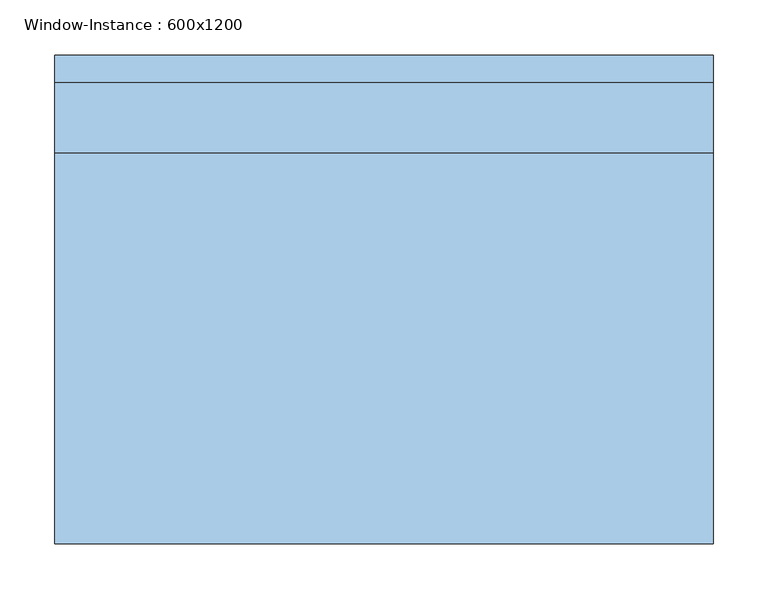
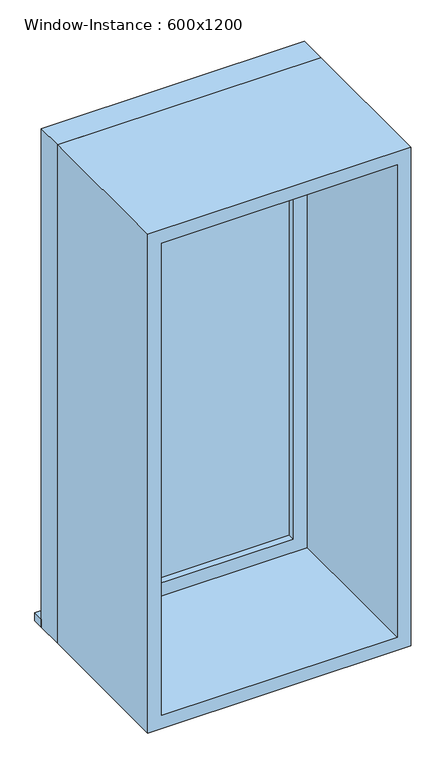
"""IFC4 building model written with IfcOpenShell, lengths in millimetres: window geometry, Window-Instance : 600x1200."""

import ifcopenshell
import ifcopenshell.guid

model = None  # the IFC model being written
_history = None  # IfcOwnerHistory: only IFC2X3 demands one
_inside = {}  # id of a spatial element -> (the spatial element, [elements in it])
_under = {}  # id of a project, library or spatial element -> (it, [spatial elements below it])
_declared = {}  # id of a project -> (the project, [libraries it declares])
_typed = {}  # id of a type object -> (the type object, [elements of that type])
_made_of = {}  # id of a material, layer set ... -> (it, [elements and type objects made of it])


def new_model(schema):
    """Start an empty IFC model of exactly this schema.

    Asked for "IFC4X3", IfcOpenShell would pick the latest addendum, in which some entities
    have other attributes; the version numbers below select the first issue.
    IFC2X3 requires an IfcOwnerHistory on every rooted entity: one is made here for all.
    """
    global model, _history
    if schema == "IFC4X3":
        model = ifcopenshell.file(schema_version=(4, 3, 0, 0))
    else:
        model = ifcopenshell.file(schema=schema)
    _inside.clear()
    _under.clear()
    _declared.clear()
    _typed.clear()
    _made_of.clear()
    _history = None
    if model.schema == "IFC2X3":
        org = make("IfcOrganization", Name="unknown")
        user = make(
            "IfcPersonAndOrganization",
            ThePerson=make("IfcPerson", FamilyName="unknown"),
            TheOrganization=org,
        )
        app = make(
            "IfcApplication",
            ApplicationDeveloper=org,
            Version="unknown",
            ApplicationFullName="unknown",
            ApplicationIdentifier="unknown",
        )
        _history = make(
            "IfcOwnerHistory",
            OwningUser=user,
            OwningApplication=app,
            ChangeAction="ADDED",
            CreationDate=0,
        )
    return model


def make(cls, **values):
    """One entity of the class cls with the attributes given. An attribute that is None is left unset."""
    return model.create_entity(
        cls, **{name: value for name, value in values.items() if value is not None}
    )


def rooted(cls, **values):
    """An entity with a GlobalId (a new one), such as an element, a storey or a relation."""
    return make(cls, GlobalId=ifcopenshell.guid.new(), OwnerHistory=_history, **values)


def si_unit(unit_type, name, prefix=None):
    """IfcSIUnit, for example si_unit("LENGTHUNIT", "METRE", prefix="MILLI")."""
    return make("IfcSIUnit", UnitType=unit_type, Prefix=prefix, Name=name)


def assignment(units):
    """IfcUnitAssignment: the units of a project."""
    return None if units is None else make("IfcUnitAssignment", Units=units)


def point(xyz):
    """IfcCartesianPoint."""
    return None if xyz is None else make("IfcCartesianPoint", Coordinates=xyz)


def direction(xyz):
    """IfcDirection."""
    return None if xyz is None else make("IfcDirection", DirectionRatios=xyz)


def frame(location, z_axis=None, x_axis=None):
    """IfcAxis2Placement3D, a coordinate frame: its origin and axes. An axis left out is left unset."""
    return make(
        "IfcAxis2Placement3D",
        Location=point(location),
        Axis=direction(z_axis),
        RefDirection=direction(x_axis),
    )


def origin():
    """The frame at (0, 0, 0) with its axes left unset."""
    return frame((0.0, 0.0, 0.0))


def place(relative_to, where):
    """IfcLocalPlacement: puts the frame where relative to a parent placement (None: the world)."""
    return make(
        "IfcLocalPlacement", PlacementRelTo=relative_to, RelativePlacement=where
    )


def context(
    kind, dimensions, precision=None, world=None, true_north=None, identifier=None
):
    """IfcGeometricRepresentationContext, for example the 3D "Model" context."""
    return make(
        "IfcGeometricRepresentationContext",
        ContextIdentifier=identifier,
        ContextType=kind,
        CoordinateSpaceDimension=dimensions,
        Precision=precision,
        WorldCoordinateSystem=world,
        TrueNorth=true_north,
    )


def project(units=None, contexts=None):
    """IfcProject with its units and contexts."""
    return rooted(
        "IfcProject",
        Name="project",
        RepresentationContexts=contexts,
        UnitsInContext=assignment(units),
    )


def spatial(cls, under=None, at=None, **own):
    """A site, building, storey or space (cls), placed at a placement, below another one or the project."""
    s = rooted(cls, ObjectPlacement=at, **own)
    if under is not None:
        _under.setdefault(under.id(), (under, []))[1].append(s)
    return s


def polyline(points):
    """IfcPolyline through the points."""
    return make("IfcPolyline", Points=[point(p) for p in points])


def outline(outer, holes=None, kind="AREA"):
    """IfcArbitraryClosedProfileDef: a profile drawn as a closed curve; with holes, ...WithVoids."""
    if holes is None:
        return make("IfcArbitraryClosedProfileDef", ProfileType=kind, OuterCurve=outer)
    return make(
        "IfcArbitraryProfileDefWithVoids",
        ProfileType=kind,
        OuterCurve=outer,
        InnerCurves=holes,
    )


def extrude(swept, where, along, depth):
    """IfcExtrudedAreaSolid: the profile swept, set in the frame where, extruded along a direction by depth."""
    return make(
        "IfcExtrudedAreaSolid",
        SweptArea=swept,
        Position=where,
        ExtrudedDirection=direction(along),
        Depth=depth,
    )


def shape(context_of_items, identifier, shape_type, items):
    """IfcShapeRepresentation: the items that make up one representation, for example the "Body"."""
    return make(
        "IfcShapeRepresentation",
        ContextOfItems=context_of_items,
        RepresentationIdentifier=identifier,
        RepresentationType=shape_type,
        Items=items,
    )


def source(mapping_origin, context_of_items, identifier, shape_type, items):
    """IfcRepresentationMap: a shape defined once, which mapped items show again and again."""
    return make(
        "IfcRepresentationMap",
        MappingOrigin=mapping_origin,
        MappedRepresentation=shape(context_of_items, identifier, shape_type, items),
    )


def transform(
    local_origin,
    x_axis=None,
    y_axis=None,
    z_axis=None,
    scale=None,
    scale2=None,
    scale3=None,
    uniform=True,
):
    """IfcCartesianTransformationOperator3D, or its non-uniform kind. x_axis, y_axis, z_axis: its Axis1, 2, 3."""
    if uniform:
        return make(
            "IfcCartesianTransformationOperator3D",
            Axis1=direction(x_axis),
            Axis2=direction(y_axis),
            LocalOrigin=point(local_origin),
            Scale=scale,
            Axis3=direction(z_axis),
        )
    return make(
        "IfcCartesianTransformationOperator3DnonUniform",
        Axis1=direction(x_axis),
        Axis2=direction(y_axis),
        LocalOrigin=point(local_origin),
        Scale=scale,
        Axis3=direction(z_axis),
        Scale2=scale2,
        Scale3=scale3,
    )


def mapped(mapping_source, mapping_target):
    """IfcMappedItem: shows the shape of a source again, moved by a transform."""
    return make(
        "IfcMappedItem", MappingSource=mapping_source, MappingTarget=mapping_target
    )


def made_of(thing, what):
    """Note that an element or type object is made of a material, layer set ...; save() writes the relation."""
    if what is not None:
        _made_of.setdefault(what.id(), (what, []))[1].append(thing)
    return thing


def element(
    cls,
    number,
    at=None,
    inside=None,
    cuts=None,
    type_object=None,
    material=None,
    context=None,
    identifier="Body",
    shape_type=None,
    held_by="IfcProductDefinitionShape",
    body=None,
    shapes=None,
    **own,
):
    """One element of the class cls, such as IfcWall. Its Tag is "e" and its number.

    at: its placement. inside: the storey or other place that contains it. cuts: it is an
    opening in that element (IfcRelVoidsElement). A single representation is given by context,
    identifier, shape_type and body (its items); several are given by shapes. held_by: the class
    of the entity that holds the representations. save() writes the other relations.
    """
    e = rooted(cls, Tag="e%d" % number, ObjectPlacement=at, **own)
    if body is not None:
        shapes = [shape(context, identifier, shape_type, body)]
    if shapes is not None:
        e.Representation = make(held_by, Representations=shapes)
    if inside is not None:
        _inside.setdefault(inside.id(), (inside, []))[1].append(e)
    if cuts is not None:
        rooted(
            "IfcRelVoidsElement", RelatingBuildingElement=cuts, RelatedOpeningElement=e
        )
    if type_object is not None:
        _typed.setdefault(type_object.id(), (type_object, []))[1].append(e)
    return made_of(e, material)


def aggregate(whole, parts):
    """IfcRelAggregates: a whole, such as a stair, and the parts it consists of."""
    return rooted("IfcRelAggregates", RelatingObject=whole, RelatedObjects=parts)


def save(model, path):
    """Write the relations noted so far, then the file.

    IfcRelAggregates (storeys below a building ...), IfcRelContainedInSpatialStructure (elements
    in a storey), IfcRelDefinesByType, IfcRelAssociatesMaterial and IfcRelDeclares: one each for
    every whole, place, type object, material and project.
    """
    for whole, parts in _under.values():
        aggregate(whole, parts)
    for where, things in _inside.values():
        rooted(
            "IfcRelContainedInSpatialStructure",
            RelatedElements=things,
            RelatingStructure=where,
        )
    for kind, things in _typed.values():
        rooted("IfcRelDefinesByType", RelatedObjects=things, RelatingType=kind)
    for what, things in _made_of.values():
        rooted("IfcRelAssociatesMaterial", RelatedObjects=things, RelatingMaterial=what)
    for by, libraries in _declared.values():
        rooted("IfcRelDeclares", RelatingContext=by, RelatedDefinitions=libraries)
    model.write(path)


def window_instance_600x1200_5a3ea86a(model_context):
    return source(origin(), model_context, "Body", "SweptSolid", [
        extrude(outline(polyline([(-338.1, 235.4), (261.9, 235.4), (261.9, 210.0), (-338.1, 210.0), (-338.1, 235.4)])), frame((0.0, 0.0, 900.0), z_axis=(0.0, 0.0, 1.0), x_axis=(1.0, 0.0, 0.0)), (0.0, 0.0, 1.0), 19.05),
        extrude(outline(polyline([(198.4, 161.425), (-274.6, 161.425), (-274.6, 174.125), (198.4, 174.125), (198.4, 161.425)])), frame((0.0, 0.0, 963.5), z_axis=(0.0, 0.0, 1.0), x_axis=(1.0, 0.0, 0.0)), (0.0, 0.0, 1.0), 1073.0),
        extrude(outline(polyline([(2080.95, -319.05), (919.05, -319.05), (919.05, 242.85), (2080.95, 242.85), (2080.95, -319.05)]), holes=[polyline([(2036.5, -274.6), (2036.5, 198.4), (963.5, 198.4), (963.5, -274.6), (2036.5, -274.6)])]), frame((0.0, 145.55, 0.0), z_axis=(0.0, 1.0, 0.0), x_axis=(0.0, 0.0, 1.0)), (0.0, 0.0, 1.0), 44.45),
        extrude(outline(polyline([(2100.0, -338.1), (900.0, -338.1), (900.0, 261.9), (2100.0, 261.9), (2100.0, -338.1)]), holes=[polyline([(2068.25, -306.35), (2068.25, 230.15), (931.75, 230.15), (931.75, -306.35), (2068.25, -306.35)])]), frame((0.0, -210.0, 0.0), z_axis=(0.0, 1.0, 0.0), x_axis=(0.0, 0.0, 1.0)), (0.0, 0.0, 1.0), 355.55),
        extrude(outline(polyline([(2100.0, 261.9), (2100.0, -338.1), (900.0, -338.1), (900.0, 261.9), (2100.0, 261.9)]), holes=[polyline([(2080.95, 242.85), (919.05, 242.85), (919.05, -319.05), (2080.95, -319.05), (2080.95, 242.85)])]), frame((0.0, 145.55, 0.0), z_axis=(0.0, 1.0, 0.0), x_axis=(0.0, 0.0, 1.0)), (0.0, 0.0, 1.0), 64.45),
    ])


if __name__ == "__main__":
    model = new_model("IFC4")
    model_context = context("Model", 3, world=origin())
    ifc_project = project(units=[si_unit("LENGTHUNIT", "METRE", prefix="MILLI")], contexts=[model_context])
    site = spatial("IfcSite", under=ifc_project)
    building = spatial("IfcBuilding", under=site)
    placement = place(None, origin())
    window_instance_600x1200_shape = window_instance_600x1200_5a3ea86a(model_context)
    element("IfcWindow", 1, ObjectType="Window-Instance : 600x1200", at=placement, inside=building, context=model_context, shape_type="MappedRepresentation", body=[
        mapped(window_instance_600x1200_shape, transform((0.0, 0.0, 0.0), x_axis=(1.0, 0.0, 0.0), y_axis=(0.0, 1.0, 0.0), z_axis=(0.0, 0.0, 1.0))),
    ])
    save(model, "model.ifc")

# Revit data of these elements
# Type "Window-Instance : 600x1200"
#   Type Mark = "7"
#   Construction Type Id = "GSP4R"
#   Assembly Code = "B2020100"
#   Analytic Construction = "1/8 in Pilkington single glazing"
#   Visual Light Transmittance = 0.9
#   Thermal Resistance (R) = 0.149095 (m²·K)/W
#   Solar Heat Gain Coefficient = 0.86
#   Heat Transfer Coefficient (U) = 6.70716 W/(m²·K)
#   Height [instance default] = 1200 mm
#   Default Sill Height = 900 mm
#   Width [instance default] = 600 mm
#   Window Inset = 20 mm
#   Glass Pane Material = WW-EC-GL-Storefront
#   Sash Material = WW-EC-RGB-White
#   Wall Closure = (empty or 0)
# Element 1 (IfcWindow, "Window-Instance : 600x1200")
#   Materials on its faces: "WW-EC-RGB-White", "WW-EC-GL-Storefront"
# Materials
#   "WW-EC-GL-Storefront": class "Glass", colour RGB 236 240 239, transparency 0.85, Description = "Storefront Glass", Cost = 0
#   "WW-EC-RGB-White": class "Generic", colour RGB 255 255 255, transparency 0, Comments = "If region requests off-white, swith asset color to RGB 231-228-220", Description = "Generic Color", Cost = 0
